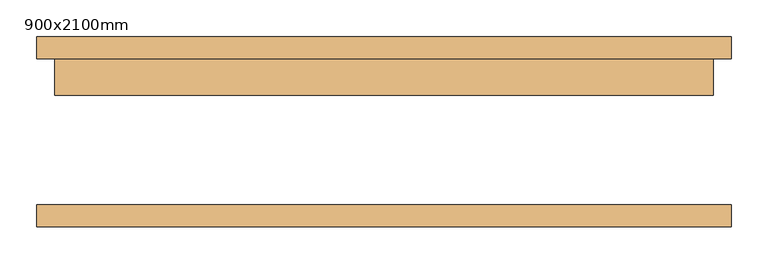
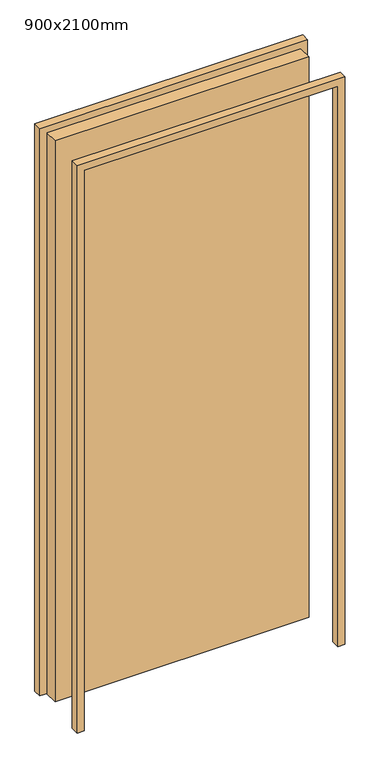
"""IFC4 building model written with IfcOpenShell, lengths in millimetres: door geometry, WWm-SingleSolid-Flush : 900x2100mm."""

from ifc_helpers import new_model, si_unit, frame, origin, origin_with_axes, place, context, project, spatial, polyline, outline, extrude, source, transform, mapped, element, save


def door_900x2100mm_0e591ed2(model_context):
    return source(origin(), model_context, "Body", "SweptSolid", [
        extrude(outline(polyline([(2125.0, -475.0), (0.0, -475.0), (0.0, -450.0), (2100.0, -450.0), (2100.0, 450.0), (0.0, 450.0), (0.0, 475.0), (2125.0, 475.0), (2125.0, -475.0)])), frame((0.0, 100.0, 0.0), z_axis=(0.0, 1.0, 0.0), x_axis=(0.0, 0.0, 1.0)), (0.0, 0.0, 1.0), 30.0),
        extrude(outline(polyline([(2125.0, 475.0), (2125.0, -475.0), (0.0, -475.0), (0.0, -450.0), (2100.0, -450.0), (2100.0, 450.0), (0.0, 450.0), (0.0, 475.0), (2125.0, 475.0)])), frame((0.0, -130.0, 0.0), z_axis=(0.0, 1.0, 0.0), x_axis=(0.0, 0.0, 1.0)), (0.0, 0.0, 1.0), 30.0),
        extrude(outline(polyline([(450.0, 50.0), (-450.0, 50.0), (-450.0, 100.0), (450.0, 100.0), (450.0, 50.0)])), origin_with_axes(), (0.0, 0.0, 1.0), 2100.0),
    ])


if __name__ == "__main__":
    model = new_model("IFC4")
    model_context = context("Model", 3, world=origin())
    ifc_project = project(units=[si_unit("LENGTHUNIT", "METRE", prefix="MILLI")], contexts=[model_context])
    site = spatial("IfcSite", under=ifc_project)
    building = spatial("IfcBuilding", under=site)
    placement = place(None, origin())
    door_900x2100mm_shape = door_900x2100mm_0e591ed2(model_context)
    element("IfcDoor", 1, ObjectType="WWm-SingleSolid-Flush : 900x2100mm", at=placement, inside=building, context=model_context, shape_type="MappedRepresentation", body=[
        mapped(door_900x2100mm_shape, transform((0.0, 0.0, 0.0), x_axis=(1.0, 0.0, 0.0), y_axis=(0.0, 1.0, 0.0), z_axis=(0.0, 0.0, 1.0))),
    ])
    save(model, "model.ifc")

# Revit data of these elements
# Type "WWm-SingleSolid-Flush : 900x2100mm"
#   Type Mark = "EX1-52"
#   Construction Type Id = "MDOOR"
#   Assembly Code = "C1020"
#   Analytic Construction = "Metal"
#   Thickness = 50 mm
#   Thermal Resistance (R) = 0.270117 (m²·K)/W
#   Heat Transfer Coefficient (U) = 3.7021 W/(m²·K)
#   Height = 2100 mm
#   Trim Projection Ext = 30 mm
#   Trim Projection Int = 30 mm
#   Trim Width = 25 mm
#   Width = 900 mm
#   Not 90 Degree [instance default] = no
#   90 Degree [instance default] = yes
#   Door Material = WW-EC-RGB-White
#   Frame Material = WW-EC-RGB-White
#   Visual Light Transmittance = 0
#   Solar Heat Gain Coefficient = 0
#   Function = (empty or 0)
#   Wall Closure = (empty or 0)
# Element 1 (IfcDoor, "WWm-SingleSolid-Flush : 900x2100mm")
#   Materials on its faces: "WW-EC-RGB-White"
# Materials
#   "WW-EC-RGB-White": class "Generic", colour RGB 255 255 255, transparency 0, Comments = "If region requests off-white, swith asset color to RGB 231-228-220", Description = "Generic Color", Cost = 0
